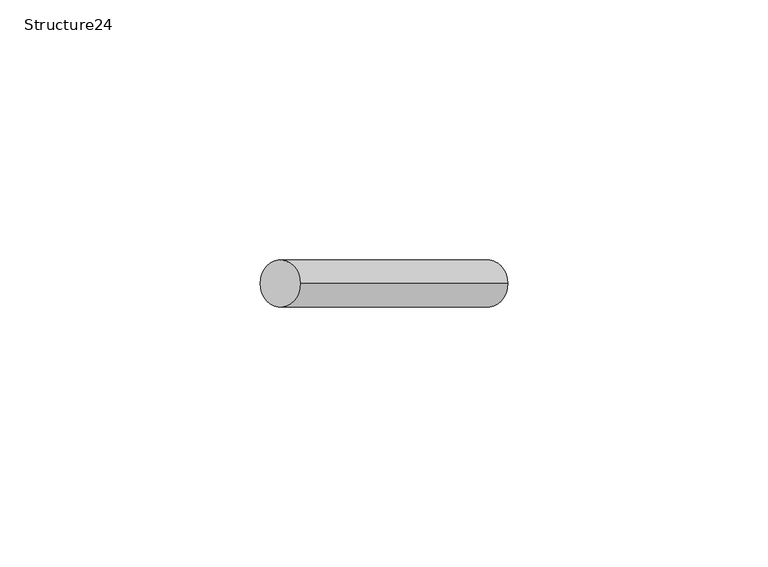
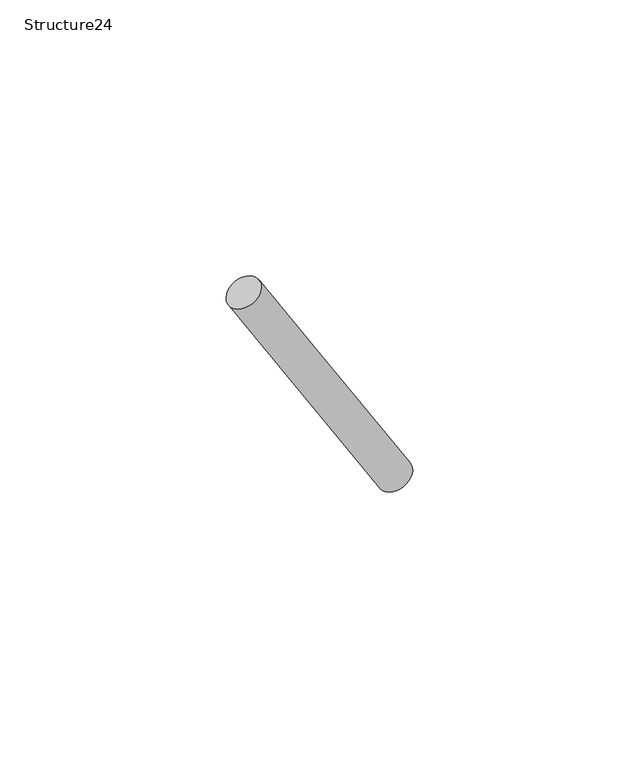
"""IFC4 building model written with IfcOpenShell, lengths in millimetres: proxy geometry, Structure24 : Structure668217152."""

from ifc_helpers import new_model, si_unit, point, frame, frame_2d, origin, place, context, project, spatial, circle_curve, trimmed, segment, composite_curve, outline, extrude, source, transform, mapped, element, save


def structure24_43e84b46(model_context):
    return source(origin(), model_context, "Body", "SweptSolid", [
        extrude(outline(composite_curve([segment(trimmed(circle_curve(frame_2d((0.0, -4.5217366)), 4.5217366), [point((0.0, -9.0434732))], [point((0.0, 0.0))], False, "CARTESIAN"), True, "CONTINUOUS"), segment(trimmed(circle_curve(frame_2d((0.0, -4.5217366)), 4.5217366), [point((0.0, 0.0))], [point((0.0, -9.0434732))], False, "CARTESIAN"), True, "CONTINUOUS")], self_intersect=False)), frame((9860.4613501, 1851.7391858, 40896.850645), z_axis=(-0.523016219738758, 0.0, 0.8523227287185172), x_axis=(0.0, -1.0, 0.0)), (0.0, 0.0, 1.0), 76.2),
    ])


if __name__ == "__main__":
    model = new_model("IFC4")
    model_context = context("Model", 3, world=origin())
    ifc_project = project(units=[si_unit("LENGTHUNIT", "METRE", prefix="MILLI")], contexts=[model_context])
    site = spatial("IfcSite", under=ifc_project)
    building = spatial("IfcBuilding", under=site)
    placement = place(None, origin())
    structure24_shape = structure24_43e84b46(model_context)
    element("IfcBuildingElementProxy", 1, Name="Structure24 : Structure668217152", ObjectType="Structure24 : Structure668217152", at=placement, inside=building, context=model_context, shape_type="MappedRepresentation", body=[
        mapped(structure24_shape, transform((0.0, 0.0, 0.0), x_axis=(1.0, 0.0, 0.0), y_axis=(0.0, 1.0, 0.0), z_axis=(0.0, 0.0, 1.0))),
    ])
    save(model, "model.ifc")

# Revit data of these elements
# Type "Structure24 : Structure668217152"
#   NameOverride = "Structure668217152"
# Element 1 (IfcBuildingElementProxy, "Structure24 : Structure668217152")
#   Materials on its faces: "1.5\" DIA. STAINLESS STEEL RAILING"
# Materials
#   "1.5\" DIA. STAINLESS STEEL RAILING": class "Unassigned", colour RGB 128 128 128, transparency 0, Cost = 0
